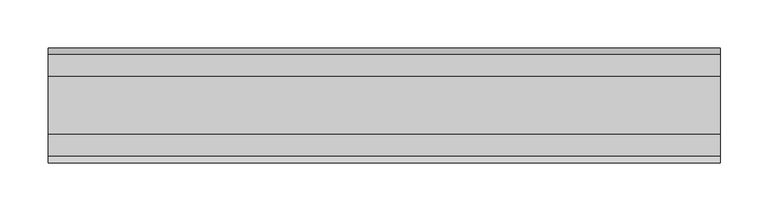
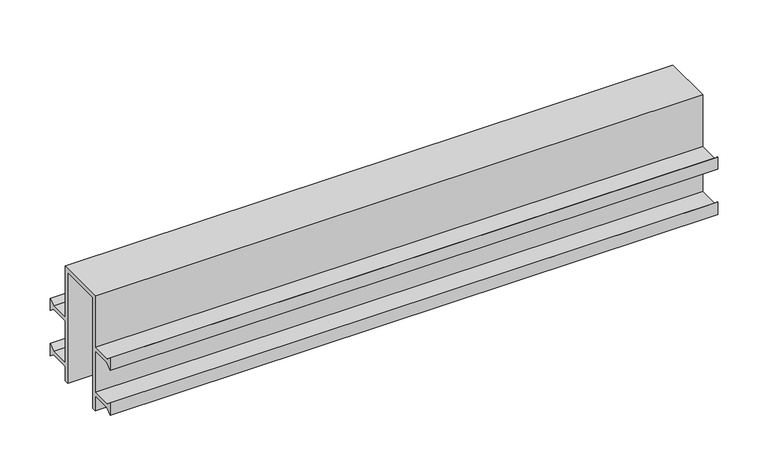
"""IFC4 building model written with IfcOpenShell, lengths in millimetres: proxy geometry, TN_Гидрошпонка ТН Фундамент : Гидрошпонка ТН Фундамент ДШП-В-50."""

from ifc_helpers import new_model, si_unit, frame, origin, place, context, project, spatial, polyline, outline, extrude, source, transform, mapped, element, save


def specialty_equipment_c495371f(model_context):
    return source(origin(), model_context, "Body", "SweptSolid", [
        extrude(outline(polyline([(25.0, -5.0), (-25.0, -5.0), (-25.0, -140.0), (-30.0, -140.0), (-30.0, -122.1), (-53.120566, -122.1), (-60.0, -127.5), (-60.0, -112.5), (-53.120566, -117.9), (-30.0, -117.9), (-30.0, -67.1), (-53.120566, -67.1), (-60.0, -72.5), (-60.0, -57.5), (-53.120566, -62.9), (-30.0, -62.9), (-30.0, 0.0), (30.0, 0.0), (30.0, -62.9), (53.120566, -62.9), (60.0, -57.5), (60.0, -72.5), (53.120566, -67.1), (30.0, -67.1), (30.0, -117.9), (53.120566, -117.9), (60.0, -112.5), (60.0, -127.5), (53.120566, -122.1), (30.0, -122.1), (30.0, -140.0), (25.0, -140.0), (25.0, -5.0)])), frame((0.0, 0.0, 0.0), z_axis=(1.0, 0.0, 0.0), x_axis=(0.0, 1.0, 0.0)), (0.0, 0.0, 1.0), 700.0),
    ])


if __name__ == "__main__":
    model = new_model("IFC4")
    model_context = context("Model", 3, world=origin())
    ifc_project = project(units=[si_unit("LENGTHUNIT", "METRE", prefix="MILLI")], contexts=[model_context])
    site = spatial("IfcSite", under=ifc_project)
    building = spatial("IfcBuilding", under=site)
    placement = place(None, origin())
    specialty_equipment_shape = specialty_equipment_c495371f(model_context)
    element("IfcBuildingElementProxy", 1, Name="TN_Гидрошпонка ТН Фундамент : Гидрошпонка ТН Фундамент ДШП-В-50", ObjectType="TN_Гидрошпонка ТН Фундамент : Гидрошпонка ТН Фундамент ДШП-В-50", at=placement, inside=building, context=model_context, shape_type="MappedRepresentation", body=[
        mapped(specialty_equipment_shape, transform((0.0, 0.0, 0.0), x_axis=(1.0, 0.0, 0.0), y_axis=(0.0, 1.0, 0.0), z_axis=(0.0, 0.0, 1.0))),
    ])
    save(model, "model.ifc")

# Revit data of these elements
# Type "TN_Гидрошпонка ТН Фундамент : Гидрошпонка ТН Фундамент ДШП-В-50"
#   Description = "Внутренние П-образные гидроизоляционные шпонки ТН Фундамент ДШП-В представляют собой профилированную ленту, изготовленную из пластифицированного поливинилхлорида методом экструзии."
#   Type Comments = "п.м."
#   Manufacturer = "ТехноНИКОЛЬ"
#   URL = "https://nav.tn.ru/catalog/gidroizolyatsiya/komplektatsiya-dlya-gidroizolyatsii/gidroshponki-tekhnonikol-fundament-dshp-v/"
#   ADSK_Примечание = ""
#   ADSK_Обозначение [instance default] = "ТехноНИКОЛЬ"
#   ADSK_Наименование = "Гидрошпонка ТН Фундамент ДШП-В-50"
#   ADSK_Масса_Текст = ""
#   ADSK_Марка = ""
#   ADSK_Код изделия = "72231"
#   ADSK_Завод-изготовитель [instance default] = "ТехноНИКОЛЬ"
#   ADSK_Единица измерения [instance default] = "п.м."
#   ADSK_Группирование = "Гидрошпонки"
#   ADSK_URL страницы изделия = "https://nav.tn.ru/catalog/gidroizolyatsiya/komplektatsiya-dlya-gidroizolyatsii/gidroshponki-tekhnonikol-fundament-dshp-v/"
#   ADSK_URL документации изделия = "https://nav.tn.ru/upload/iblock/bef/50ps2dij0orvk11owm0y8tn3vby3otsm/Tekhlist-7.405_Gidroshponki_TN_Fundament_DSHP_V_RU_ru.pdf"
#   built-in parameter 1001306 [instance default] = 3.28084 (stored number, unit not read)
#   ADSK_Размер_Длина [instance default] = 1000 mm
#   ADSK_Количество [instance default] = 1
#   Гидрошпонка ТН Фундамент ТШ-Н-210 = no
#   Гидрошпонка ТН Фундамент ДШП-В-50 = yes
#   Гидрошпонка ТН Фундамент ДШП-В-20 = no
#   Гидрошпонка ТН Фундамент ДШ-В-280 = no
#   Гидрошпонка ТН Фундамент ДШ-В-250 = no
#   Гидрошпонка ТН Фундамент ТШ-В-250 = no
#   Гидрошпонка ТН Фундамент ТПС-В 140-1 = no
#   Гидрошпонка ТН Фундамент ДШ-Н-280 = no
#   Гидрошпонка ТН Фундамент ДШ-Н-250 = no
#   Гидрошпонка ТН Фундамент ТПС-В 100-2 = no
#   Гидрошпонка ТН Фундамент ТШ-Н-250 = no
#   Гидрошпонка ТН Фундамент ТШ-В-210 = no
#   Материал = TN_ПВХ_Черный
#   Default Elevation = 0
# Element 1 (IfcBuildingElementProxy, "TN_Гидрошпонка ТН Фундамент : Гидрошпонка ТН Фундамент ДШП-В-50")
#   built-in parameter 1001306 = 2.29659 (stored number, unit not read)
#   ADSK_Размер_Длина = 700 mm
#   ADSK_Количество = 0.7
#   Materials on its faces: "TN_ПВХ_Черный"
# Materials
#   "TN_ПВХ_Черный": class "Типовые", colour RGB 48 48 48, transparency 0, Cost = 0
